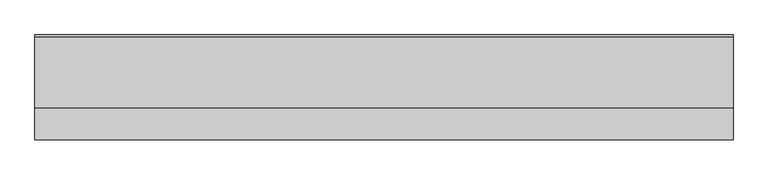
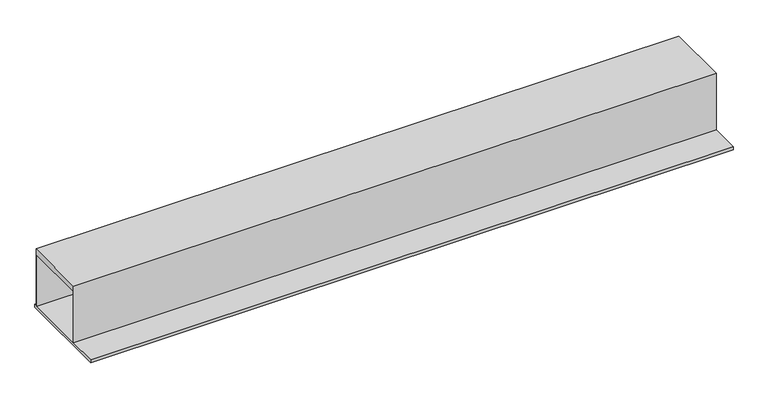
"""IFC4 building model written with IfcOpenShell, lengths in millimetres: beam geometry, NLRS_28_SF_LIB_stalen ligger THQ-AV-CWV-MMBS-SRP_gen_rsf : stalen ligger_gen__PET 280x6-290x30-450x15."""

from ifc_helpers import new_model, si_unit, frame, origin, place, context, project, spatial, polyline, outline, extrude, source, transform, mapped, element, save


def beam_bc03ea60(model_context):
    return source(origin(), model_context, "Body", "SweptSolid", [
        extrude(outline(polyline([(-139.5, 280.0), (162.5, 280.0), (162.5, 0.0), (172.5, 0.0), (172.5, -15.0), (-277.5, -15.0), (-277.5, 0.0), (-139.5, 0.0), (-139.5, 280.0)]), holes=[polyline([(-133.5, 0.0), (156.5, 0.0), (156.5, 250.0), (-133.5, 250.0), (-133.5, 0.0)])]), frame((-1499.9999994, 0.0, 0.0), z_axis=(1.0, 0.0, 0.0), x_axis=(0.0, 1.0, 0.0)), (0.0, 0.0, 1.0), 2999.9999988),
    ])


if __name__ == "__main__":
    model = new_model("IFC4")
    model_context = context("Model", 3, world=origin())
    ifc_project = project(units=[si_unit("LENGTHUNIT", "METRE", prefix="MILLI")], contexts=[model_context])
    site = spatial("IfcSite", under=ifc_project)
    building = spatial("IfcBuilding", under=site)
    placement = place(None, origin())
    beam_shape = beam_bc03ea60(model_context)
    element("IfcBeam", 1, ObjectType="NLRS_28_SF_LIB_stalen ligger THQ-AV-CWV-MMBS-SRP_gen_rsf : stalen ligger_gen__PET 280x6-290x30-450x15", at=placement, inside=building, context=model_context, shape_type="MappedRepresentation", body=[
        mapped(beam_shape, transform((0.0, 0.0, 0.0), x_axis=(1.0, 0.0, 0.0), y_axis=(0.0, 1.0, 0.0), z_axis=(0.0, 0.0, 1.0))),
    ])
    save(model, "model.ifc")

# Revit data of these elements
# Type "NLRS_28_SF_LIB_stalen ligger THQ-AV-CWV-MMBS-SRP_gen_rsf : stalen ligger_gen__PET 280x6-290x30-450x15"
#   Type IfcGUID = "0zo1UjqZ91lRsfCKsOOaAF"
#   IfcExportAs = "IfcBeamType"
#   Type Comments = "PET 280x6-290x30-450x15"
#   Model = " "
#   Manufacturer = " "
#   Fire Rating = " "
#   Description = "stalen ligger PET 280x6-290x30-450x15"
#   Assembly Code = "28.11"
#   tw = 6 mm
#   tu = 15 mm
#   to = 30 mm
#   h = 280 mm
#   bu = 450 mm
#   bo = 290 mm
#   NLRS_C_lengte [instance default] = 1500 mm
#   Length [instance default] = 1500 mm
#   RSF_C_vullen_met_beton [instance default] = no
#   RSF_C_petligger = yes
#   RSF_C_hoedligger = no
#   Structural Material = NLRS_h2_staal_gen_rsf
#   Keynote = ""
# Element 1 (IfcBeam, "NLRS_28_SF_LIB_stalen ligger THQ-AV-CWV-MMBS-SRP_gen_rsf : stalen ligger_gen__PET 280x6-290x30-450x15")
#   NLRS_C_lengte = 3000 mm
#   Materials on its faces: "NLRS_h2_staal_gen_rsf"
# Materials
#   "NLRS_h2_staal_gen_rsf": class "H - Metaal", colour RGB 189 187 185, transparency 0, Keynote = "h2", Manufacturer = "Revit Standards Foundation", URL = "www.revitstandards.org", Description = "staal", Cost = 0
